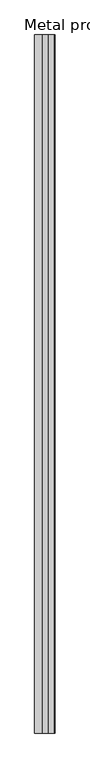
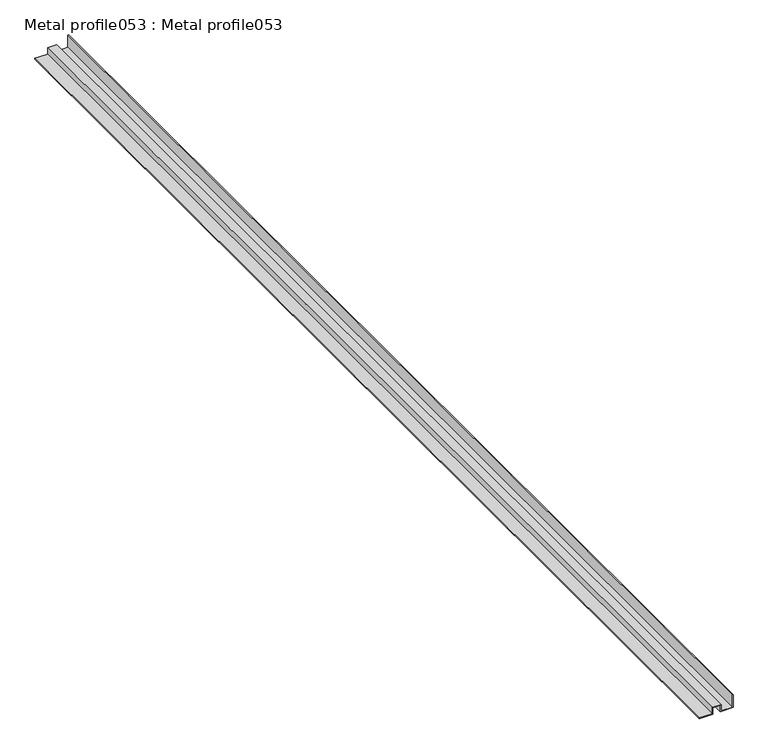
"""IFC4 building model written with IfcOpenShell, lengths in millimetres: proxy geometry, Metal profile053 : Metal profile053."""

from ifc_helpers import new_model, si_unit, frame, origin, place, context, project, spatial, polyline, outline, extrude, source, transform, mapped, element, save


def metal_profile053_metal_profile053_87e07942(model_context):
    return source(origin(), model_context, "Body", "SweptSolid", [
        extrude(outline(polyline([(39543.8875708, -4375.3289163), (39567.6883323, -4375.3289163), (39567.6883323, -4376.6089163), (39545.1675708, -4376.6089163), (39545.1675708, -4396.2739163), (39556.5975708, -4396.2739163), (39556.5975708, -4411.5339163), (39545.1675708, -4411.5339163), (39545.1675708, -4433.9671002), (39543.8875708, -4433.9671002), (39543.8875708, -4410.2539163), (39555.3175708, -4410.2539163), (39555.3175708, -4397.5539163), (39543.8875708, -4397.5539163), (39543.8875708, -4375.3289163)])), frame((0.0, -1052.8906574, 0.0), z_axis=(0.0, 1.0, 0.0), x_axis=(0.0, 0.0, 1.0)), (0.0, 0.0, 1.0), 2000.0),
    ])


if __name__ == "__main__":
    model = new_model("IFC4")
    model_context = context("Model", 3, world=origin())
    ifc_project = project(units=[si_unit("LENGTHUNIT", "METRE", prefix="MILLI")], contexts=[model_context])
    site = spatial("IfcSite", under=ifc_project)
    building = spatial("IfcBuilding", under=site)
    placement = place(None, origin())
    metal_profile053_metal_profile053_shape = metal_profile053_metal_profile053_87e07942(model_context)
    element("IfcBuildingElementProxy", 1, Name="Metal profile053 : Metal profile053", ObjectType="Metal profile053 : Metal profile053", at=placement, inside=building, context=model_context, shape_type="MappedRepresentation", body=[
        mapped(metal_profile053_metal_profile053_shape, transform((0.0, 0.0, 0.0), x_axis=(1.0, 0.0, 0.0), y_axis=(0.0, 1.0, 0.0), z_axis=(0.0, 0.0, 1.0))),
    ])
    save(model, "model.ifc")

# Revit data of these elements
# Type "Metal profile053 : Metal profile053"
#   NameOverride = "Metal profile053"
# Element 1 (IfcBuildingElementProxy, "Metal profile053 : Metal profile053")
#   Materials on its faces: "16 GA. COPPER SOFFIT DRIP SCREED"
# Materials
#   "16 GA. COPPER SOFFIT DRIP SCREED": class "Unassigned", colour RGB 255 217 0, transparency 0
